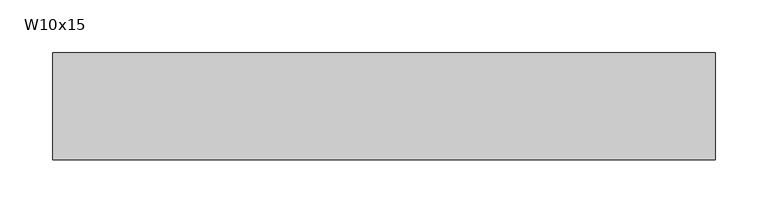
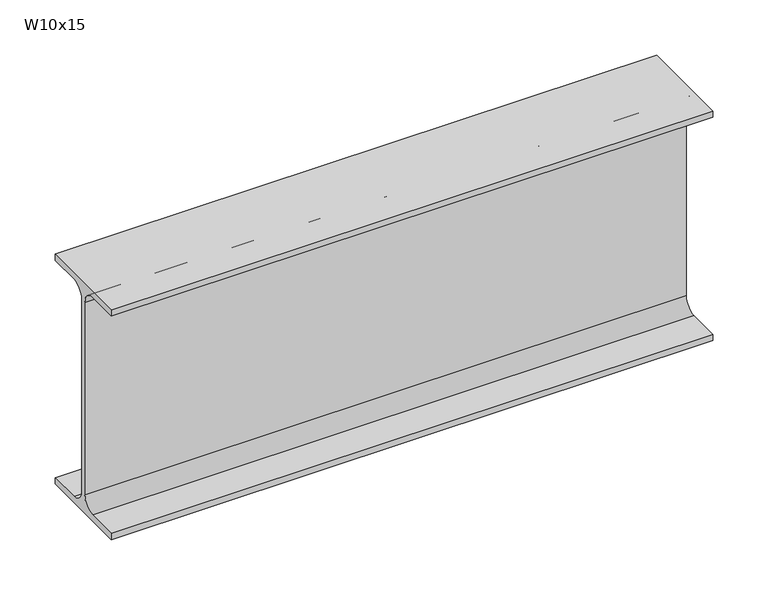
"""IFC4 building model written with IfcOpenShell, lengths in millimetres: beam geometry, RME W-Wide Flange : W10x15."""

from ifc_helpers import new_model, si_unit, point, frame, frame_2d, origin, place, context, project, spatial, polyline, circle_curve, trimmed, segment, composite_curve, outline, extrude, source, transform, mapped, element, save


def w10x15_8f499c97(model_context):
    return source(origin(), model_context, "Body", "SweptSolid", [
        extrude(outline(composite_curve([segment(polyline([(50.8, -120.142), (50.8, -127.0), (-50.8, -127.0), (-50.8, -120.142), (-16.7005, -120.142)]), True, "CONTINUOUS"), segment(trimmed(circle_curve(frame_2d((-16.7005, -106.3625)), 13.7795), [point((-16.7005, -120.142))], [point((-2.921, -106.3625))], True, "CARTESIAN"), True, "CONTINUOUS"), segment(polyline([(-2.921, -106.3625), (-2.921, 106.3625)]), True, "CONTINUOUS"), segment(trimmed(circle_curve(frame_2d((-16.7005, 106.3625)), 13.7795), [point((-2.921, 106.3625))], [point((-16.7005, 120.142))], True, "CARTESIAN"), True, "CONTINUOUS"), segment(polyline([(-16.7005, 120.142), (-50.8, 120.142), (-50.8, 127.0), (50.8, 127.0), (50.8, 120.142), (16.7005, 120.142)]), True, "CONTINUOUS"), segment(trimmed(circle_curve(frame_2d((16.7005, 106.3625)), 13.7795), [point((16.7005, 120.142))], [point((2.921, 106.3625))], True, "CARTESIAN"), True, "CONTINUOUS"), segment(polyline([(2.921, 106.3625), (2.921, -106.3625)]), True, "CONTINUOUS"), segment(trimmed(circle_curve(frame_2d((16.7005, -106.3625)), 13.7795), [point((2.921, -106.3625))], [point((16.7005, -120.142))], True, "CARTESIAN"), True, "CONTINUOUS"), segment(polyline([(16.7005, -120.142), (50.8, -120.142)]), True, "CONTINUOUS")], self_intersect=False)), frame((-241.3, 0.0, 0.0), z_axis=(1.0, 0.0, 0.0), x_axis=(0.0, 1.0, 0.0)), (0.0, 0.0, 1.0), 628.523),
    ])


if __name__ == "__main__":
    model = new_model("IFC4")
    model_context = context("Model", 3, world=origin())
    ifc_project = project(units=[si_unit("LENGTHUNIT", "METRE", prefix="MILLI")], contexts=[model_context])
    site = spatial("IfcSite", under=ifc_project)
    building = spatial("IfcBuilding", under=site)
    placement = place(None, origin())
    w10x15_shape = w10x15_8f499c97(model_context)
    element("IfcBeam", 1, ObjectType="RME W-Wide Flange : W10x15", at=placement, inside=building, context=model_context, shape_type="MappedRepresentation", body=[
        mapped(w10x15_shape, transform((0.0, 0.0, 0.0), x_axis=(1.0, 0.0, 0.0), y_axis=(0.0, 1.0, 0.0), z_axis=(0.0, 0.0, 1.0))),
    ])
    save(model, "model.ifc")

# Revit data of these elements
# Type "RME W-Wide Flange : W10x15"
#   WELD P [instance default] = ""
#   WELD LE [instance default] = ""
#   WELD D [instance default] = ""
#   TOP SECTION SIZE [instance default] = ""
#   TOP SECTION LENGTH [instance default] = ""
#   REMARKS [instance default] = ""
#   REINF TYPE [instance default] = ""
#   Nominal Size = "W24"
#   End Bearing Capacity [instance default] = ""
#   BOT SECTION SIZE [instance default] = ""
#   BOT SECTION LENGTH [instance default] = ""
#   Assembly Code = "B10"
#   W = 15
#   Start Extension Calculation [instance default] = 10' - 0"
#   Start Extension [instance default] = -0' - 0 1/2"
#   End Extension Calculation [instance default] = 10' - 0"
#   End Extension [instance default] = -0' - 0 1/2"
#   Length [instance default] = 5' - 0"
#   bf = 0' - 4"
#   d = 0' - 10"
#   k = 0' - 0 13/16"
#   k2 = 0' - 0.5425"
#   tf = 0' - 0.27"
#   tw = 0' - 0.23"
#   A = 0.030625 SF
#   Structural Material [instance default] = Metal - Steel - ASTM A992
# Element 1 (IfcBeam, "RME W-Wide Flange : W10x15")
#   Length = 2' - 0"
#   Materials on its faces: "Metal - Steel - ASTM A992"
# Materials
#   "Metal - Steel - ASTM A992": class "Metal", colour RGB 255 128 0, transparency 0
